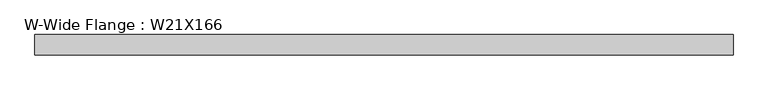
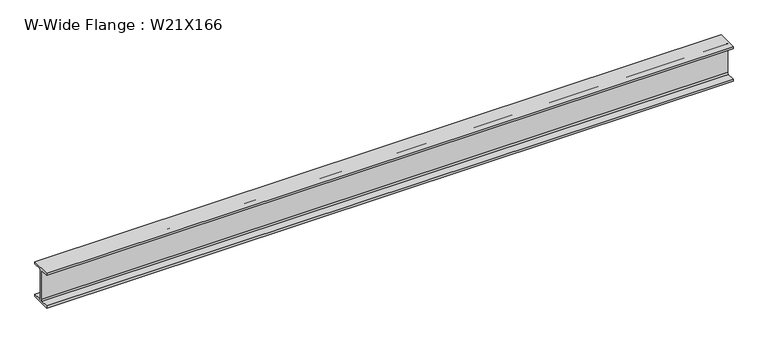
"""IFC4 building model written with IfcOpenShell, lengths in millimetres: beam geometry, W-Wide Flange : W21X166."""

import ifcopenshell
import ifcopenshell.guid

model = None  # the IFC model being written
_history = None  # IfcOwnerHistory: only IFC2X3 demands one
_inside = {}  # id of a spatial element -> (the spatial element, [elements in it])
_under = {}  # id of a project, library or spatial element -> (it, [spatial elements below it])
_declared = {}  # id of a project -> (the project, [libraries it declares])
_typed = {}  # id of a type object -> (the type object, [elements of that type])
_made_of = {}  # id of a material, layer set ... -> (it, [elements and type objects made of it])


def new_model(schema):
    """Start an empty IFC model of exactly this schema.

    Asked for "IFC4X3", IfcOpenShell would pick the latest addendum, in which some entities
    have other attributes; the version numbers below select the first issue.
    IFC2X3 requires an IfcOwnerHistory on every rooted entity: one is made here for all.
    """
    global model, _history
    if schema == "IFC4X3":
        model = ifcopenshell.file(schema_version=(4, 3, 0, 0))
    else:
        model = ifcopenshell.file(schema=schema)
    _inside.clear()
    _under.clear()
    _declared.clear()
    _typed.clear()
    _made_of.clear()
    _history = None
    if model.schema == "IFC2X3":
        org = make("IfcOrganization", Name="unknown")
        user = make(
            "IfcPersonAndOrganization",
            ThePerson=make("IfcPerson", FamilyName="unknown"),
            TheOrganization=org,
        )
        app = make(
            "IfcApplication",
            ApplicationDeveloper=org,
            Version="unknown",
            ApplicationFullName="unknown",
            ApplicationIdentifier="unknown",
        )
        _history = make(
            "IfcOwnerHistory",
            OwningUser=user,
            OwningApplication=app,
            ChangeAction="ADDED",
            CreationDate=0,
        )
    return model


def make(cls, **values):
    """One entity of the class cls with the attributes given. An attribute that is None is left unset."""
    return model.create_entity(
        cls, **{name: value for name, value in values.items() if value is not None}
    )


def rooted(cls, **values):
    """An entity with a GlobalId (a new one), such as an element, a storey or a relation."""
    return make(cls, GlobalId=ifcopenshell.guid.new(), OwnerHistory=_history, **values)


def si_unit(unit_type, name, prefix=None):
    """IfcSIUnit, for example si_unit("LENGTHUNIT", "METRE", prefix="MILLI")."""
    return make("IfcSIUnit", UnitType=unit_type, Prefix=prefix, Name=name)


def assignment(units):
    """IfcUnitAssignment: the units of a project."""
    return None if units is None else make("IfcUnitAssignment", Units=units)


def point(xyz):
    """IfcCartesianPoint."""
    return None if xyz is None else make("IfcCartesianPoint", Coordinates=xyz)


def direction(xyz):
    """IfcDirection."""
    return None if xyz is None else make("IfcDirection", DirectionRatios=xyz)


def frame(location, z_axis=None, x_axis=None):
    """IfcAxis2Placement3D, a coordinate frame: its origin and axes. An axis left out is left unset."""
    return make(
        "IfcAxis2Placement3D",
        Location=point(location),
        Axis=direction(z_axis),
        RefDirection=direction(x_axis),
    )


def frame_2d(location, x_axis=None):
    """IfcAxis2Placement2D, a coordinate frame in the plane: its origin and x axis."""
    return make(
        "IfcAxis2Placement2D", Location=point(location), RefDirection=direction(x_axis)
    )


def origin():
    """The frame at (0, 0, 0) with its axes left unset."""
    return frame((0.0, 0.0, 0.0))


def place(relative_to, where):
    """IfcLocalPlacement: puts the frame where relative to a parent placement (None: the world)."""
    return make(
        "IfcLocalPlacement", PlacementRelTo=relative_to, RelativePlacement=where
    )


def context(
    kind, dimensions, precision=None, world=None, true_north=None, identifier=None
):
    """IfcGeometricRepresentationContext, for example the 3D "Model" context."""
    return make(
        "IfcGeometricRepresentationContext",
        ContextIdentifier=identifier,
        ContextType=kind,
        CoordinateSpaceDimension=dimensions,
        Precision=precision,
        WorldCoordinateSystem=world,
        TrueNorth=true_north,
    )


def project(units=None, contexts=None):
    """IfcProject with its units and contexts."""
    return rooted(
        "IfcProject",
        Name="project",
        RepresentationContexts=contexts,
        UnitsInContext=assignment(units),
    )


def spatial(cls, under=None, at=None, **own):
    """A site, building, storey or space (cls), placed at a placement, below another one or the project."""
    s = rooted(cls, ObjectPlacement=at, **own)
    if under is not None:
        _under.setdefault(under.id(), (under, []))[1].append(s)
    return s


def polyline(points):
    """IfcPolyline through the points."""
    return make("IfcPolyline", Points=[point(p) for p in points])


def circle_curve(where, radius):
    """IfcCircle in the frame where."""
    return make("IfcCircle", Position=where, Radius=radius)


def trimmed(basis, trim1, trim2, sense, master):
    """IfcTrimmedCurve: the piece of a basis curve between two trims."""
    return make(
        "IfcTrimmedCurve",
        BasisCurve=basis,
        Trim1=trim1,
        Trim2=trim2,
        SenseAgreement=sense,
        MasterRepresentation=master,
    )


def segment(curve, same_sense, transition):
    """IfcCompositeCurveSegment."""
    return make(
        "IfcCompositeCurveSegment",
        Transition=transition,
        SameSense=same_sense,
        ParentCurve=curve,
    )


def composite_curve(segments, self_intersect=None):
    """IfcCompositeCurve: segments joined end to end."""
    return make("IfcCompositeCurve", Segments=segments, SelfIntersect=self_intersect)


def outline(outer, holes=None, kind="AREA"):
    """IfcArbitraryClosedProfileDef: a profile drawn as a closed curve; with holes, ...WithVoids."""
    if holes is None:
        return make("IfcArbitraryClosedProfileDef", ProfileType=kind, OuterCurve=outer)
    return make(
        "IfcArbitraryProfileDefWithVoids",
        ProfileType=kind,
        OuterCurve=outer,
        InnerCurves=holes,
    )


def extrude(swept, where, along, depth):
    """IfcExtrudedAreaSolid: the profile swept, set in the frame where, extruded along a direction by depth."""
    return make(
        "IfcExtrudedAreaSolid",
        SweptArea=swept,
        Position=where,
        ExtrudedDirection=direction(along),
        Depth=depth,
    )


def shape(context_of_items, identifier, shape_type, items):
    """IfcShapeRepresentation: the items that make up one representation, for example the "Body"."""
    return make(
        "IfcShapeRepresentation",
        ContextOfItems=context_of_items,
        RepresentationIdentifier=identifier,
        RepresentationType=shape_type,
        Items=items,
    )


def source(mapping_origin, context_of_items, identifier, shape_type, items):
    """IfcRepresentationMap: a shape defined once, which mapped items show again and again."""
    return make(
        "IfcRepresentationMap",
        MappingOrigin=mapping_origin,
        MappedRepresentation=shape(context_of_items, identifier, shape_type, items),
    )


def transform(
    local_origin,
    x_axis=None,
    y_axis=None,
    z_axis=None,
    scale=None,
    scale2=None,
    scale3=None,
    uniform=True,
):
    """IfcCartesianTransformationOperator3D, or its non-uniform kind. x_axis, y_axis, z_axis: its Axis1, 2, 3."""
    if uniform:
        return make(
            "IfcCartesianTransformationOperator3D",
            Axis1=direction(x_axis),
            Axis2=direction(y_axis),
            LocalOrigin=point(local_origin),
            Scale=scale,
            Axis3=direction(z_axis),
        )
    return make(
        "IfcCartesianTransformationOperator3DnonUniform",
        Axis1=direction(x_axis),
        Axis2=direction(y_axis),
        LocalOrigin=point(local_origin),
        Scale=scale,
        Axis3=direction(z_axis),
        Scale2=scale2,
        Scale3=scale3,
    )


def mapped(mapping_source, mapping_target):
    """IfcMappedItem: shows the shape of a source again, moved by a transform."""
    return make(
        "IfcMappedItem", MappingSource=mapping_source, MappingTarget=mapping_target
    )


def made_of(thing, what):
    """Note that an element or type object is made of a material, layer set ...; save() writes the relation."""
    if what is not None:
        _made_of.setdefault(what.id(), (what, []))[1].append(thing)
    return thing


def element(
    cls,
    number,
    at=None,
    inside=None,
    cuts=None,
    type_object=None,
    material=None,
    context=None,
    identifier="Body",
    shape_type=None,
    held_by="IfcProductDefinitionShape",
    body=None,
    shapes=None,
    **own,
):
    """One element of the class cls, such as IfcWall. Its Tag is "e" and its number.

    at: its placement. inside: the storey or other place that contains it. cuts: it is an
    opening in that element (IfcRelVoidsElement). A single representation is given by context,
    identifier, shape_type and body (its items); several are given by shapes. held_by: the class
    of the entity that holds the representations. save() writes the other relations.
    """
    e = rooted(cls, Tag="e%d" % number, ObjectPlacement=at, **own)
    if body is not None:
        shapes = [shape(context, identifier, shape_type, body)]
    if shapes is not None:
        e.Representation = make(held_by, Representations=shapes)
    if inside is not None:
        _inside.setdefault(inside.id(), (inside, []))[1].append(e)
    if cuts is not None:
        rooted(
            "IfcRelVoidsElement", RelatingBuildingElement=cuts, RelatedOpeningElement=e
        )
    if type_object is not None:
        _typed.setdefault(type_object.id(), (type_object, []))[1].append(e)
    return made_of(e, material)


def aggregate(whole, parts):
    """IfcRelAggregates: a whole, such as a stair, and the parts it consists of."""
    return rooted("IfcRelAggregates", RelatingObject=whole, RelatedObjects=parts)


def save(model, path):
    """Write the relations noted so far, then the file.

    IfcRelAggregates (storeys below a building ...), IfcRelContainedInSpatialStructure (elements
    in a storey), IfcRelDefinesByType, IfcRelAssociatesMaterial and IfcRelDeclares: one each for
    every whole, place, type object, material and project.
    """
    for whole, parts in _under.values():
        aggregate(whole, parts)
    for where, things in _inside.values():
        rooted(
            "IfcRelContainedInSpatialStructure",
            RelatedElements=things,
            RelatingStructure=where,
        )
    for kind, things in _typed.values():
        rooted("IfcRelDefinesByType", RelatedObjects=things, RelatingType=kind)
    for what, things in _made_of.values():
        rooted("IfcRelAssociatesMaterial", RelatedObjects=things, RelatingMaterial=what)
    for by, libraries in _declared.values():
        rooted("IfcRelDeclares", RelatingContext=by, RelatedDefinitions=libraries)
    model.write(path)


def w_wide_flange_w21x166_c5877593(model_context):
    return source(origin(), model_context, "Body", "SweptSolid", [
        extrude(outline(composite_curve([segment(polyline([(157.48, -251.206), (157.48, -285.75), (-157.48, -285.75), (-157.48, -251.206), (-32.131, -251.206)]), True, "CONTINUOUS"), segment(trimmed(circle_curve(frame_2d((-32.131, -228.6)), 22.606), [point((-32.131, -251.206))], [point((-9.525, -228.6))], True, "CARTESIAN"), True, "CONTINUOUS"), segment(polyline([(-9.525, -228.6), (-9.525, 228.6)]), True, "CONTINUOUS"), segment(trimmed(circle_curve(frame_2d((-32.131, 228.6)), 22.606), [point((-9.525, 228.6))], [point((-32.131, 251.206))], True, "CARTESIAN"), True, "CONTINUOUS"), segment(polyline([(-32.131, 251.206), (-157.48, 251.206), (-157.48, 285.75), (157.48, 285.75), (157.48, 251.206), (32.131, 251.206)]), True, "CONTINUOUS"), segment(trimmed(circle_curve(frame_2d((32.131, 228.6)), 22.606), [point((32.131, 251.206))], [point((9.525, 228.6))], True, "CARTESIAN"), True, "CONTINUOUS"), segment(polyline([(9.525, 228.6), (9.525, -228.6)]), True, "CONTINUOUS"), segment(trimmed(circle_curve(frame_2d((32.131, -228.6)), 22.606), [point((9.525, -228.6))], [point((32.131, -251.206))], True, "CARTESIAN"), True, "CONTINUOUS"), segment(polyline([(32.131, -251.206), (157.48, -251.206)]), True, "CONTINUOUS")], self_intersect=False)), frame((-5297.1995407, 0.0, 0.0), z_axis=(1.0, 0.0, 0.0), x_axis=(0.0, 1.0, 0.0)), (0.0, 0.0, 1.0), 10684.4353832),
    ])


if __name__ == "__main__":
    model = new_model("IFC4")
    model_context = context("Model", 3, world=origin())
    ifc_project = project(units=[si_unit("LENGTHUNIT", "METRE", prefix="MILLI")], contexts=[model_context])
    site = spatial("IfcSite", under=ifc_project)
    building = spatial("IfcBuilding", under=site)
    placement = place(None, origin())
    w_wide_flange_w21x166_shape = w_wide_flange_w21x166_c5877593(model_context)
    element("IfcBeam", 1, ObjectType="W-Wide Flange : W21X166", at=placement, inside=building, context=model_context, shape_type="MappedRepresentation", body=[
        mapped(w_wide_flange_w21x166_shape, transform((0.0, 0.0, 0.0), x_axis=(1.0, 0.0, 0.0), y_axis=(0.0, 1.0, 0.0), z_axis=(0.0, 0.0, 1.0))),
    ])
    save(model, "model.ifc")

# Revit data of these elements
# Type "W-Wide Flange : W21X166"
#   Assembly Code = "B10"
#   W = 166
#   Length [instance default] = 5' - 0"
#   bf = 1' - 0.4"
#   d = 1' - 10 1/2"
#   k = 0' - 2 1/4"
#   k2 = 0' - 0.89"
#   tf = 0' - 1.36"
#   tw = 0' - 0 3/4"
#   A = 0.338889 SF
#   Structural Material [instance default] = Steel ASTM A992
# Element 1 (IfcBeam, "W-Wide Flange : W21X166")
#   Structural Material = Steel
#   Materials on its faces: "Steel"
# Materials
#   "Steel ASTM A992": class "Metal", colour RGB 199 199 199, transparency 0, Description = "Structural steel 50ksi", Cost = 0
#   "Steel": class "Metal", colour RGB 118 118 114, transparency 0, Description = "Steel, mill finish", Cost = 0
